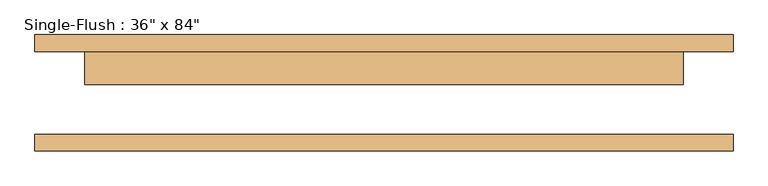
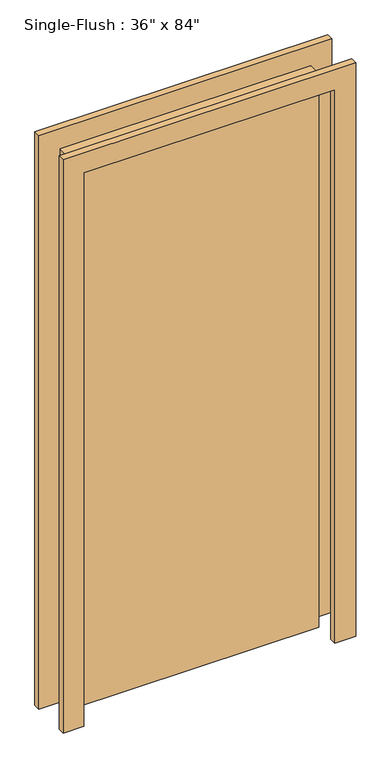
"""IFC4 building model written with IfcOpenShell, lengths in millimetres: door geometry."""

from ifc_helpers import new_model, si_unit, frame, origin, origin_with_axes, place, context, project, spatial, polyline, outline, extrude, source, transform, mapped, element, save


def door_a1797ceb(model_context):
    return source(origin(), model_context, "Body", "SweptSolid", [
        extrude(outline(polyline([(2209.8, -533.4), (0.0, -533.4), (0.0, -457.2), (2133.6, -457.2), (2133.6, 457.2), (0.0, 457.2), (0.0, 533.4), (2209.8, 533.4), (2209.8, -533.4)])), frame((0.0, 63.5, 0.0), z_axis=(0.0, 1.0, 0.0), x_axis=(0.0, 0.0, 1.0)), (0.0, 0.0, 1.0), 25.4),
        extrude(outline(polyline([(2209.8, 533.4), (2209.8, -533.4), (0.0, -533.4), (0.0, -457.2), (2133.6, -457.2), (2133.6, 457.2), (0.0, 457.2), (0.0, 533.4), (2209.8, 533.4)])), frame((0.0, -88.9, 0.0), z_axis=(0.0, 1.0, 0.0), x_axis=(0.0, 0.0, 1.0)), (0.0, 0.0, 1.0), 25.4),
        extrude(outline(polyline([(457.2, 12.7), (-457.2, 12.7), (-457.2, 63.5), (457.2, 63.5), (457.2, 12.7)])), origin_with_axes(), (0.0, 0.0, 1.0), 2133.6),
    ])


if __name__ == "__main__":
    model = new_model("IFC4")
    model_context = context("Model", 3, world=origin())
    ifc_project = project(units=[si_unit("LENGTHUNIT", "METRE", prefix="MILLI")], contexts=[model_context])
    site = spatial("IfcSite", under=ifc_project)
    building = spatial("IfcBuilding", under=site)
    placement = place(None, origin())
    door_shape = door_a1797ceb(model_context)
    element("IfcDoor", 1, ObjectType="Single-Flush : 36\" x 84\"", at=placement, inside=building, context=model_context, shape_type="MappedRepresentation", body=[
        mapped(door_shape, transform((0.0, 0.0, 0.0), x_axis=(1.0, 0.0, 0.0), y_axis=(0.0, 1.0, 0.0), z_axis=(0.0, 0.0, 1.0))),
    ])
    save(model, "model.ifc")

# Revit data of these elements
# Type "Single-Flush : 36\" x 84\""
#   Type Mark = "8"
#   Construction Type Id = "MDOOR"
#   Assembly Code = "C1020"
#   Analytic Construction = "Metal"
#   Thickness = 0' - 2"
#   Heat Transfer Coefficient (U) = 0.651978 BTU/(h·ft²·°F)
#   Height = 7' - 0"
#   Trim Projection Ext = 0' - 1"
#   Trim Projection Int = 0' - 1"
#   Trim Width = 0' - 3"
#   Width = 3' - 0"
#   Define Thermal Properties by = 1
#   Define Thermal Properties by = 1
#   Door Material = Door - Panel
#   Frame Material = Door - Frame
#   Visual Light Transmittance = 0
#   Solar Heat Gain Coefficient = 0
#   Function = (empty or 0)
#   Wall Closure = (empty or 0)
# Element 1 (IfcDoor, "Single-Flush : 36\" x 84\"")
#   Materials on its faces: "Door - Frame", "Door - Panel"
# Materials
#   "Door - Panel": class "Wood", colour RGB 210 159 95, transparency 0
#   "Door - Frame": class "Miscellaneous", colour RGB 118 70 51, transparency 0
